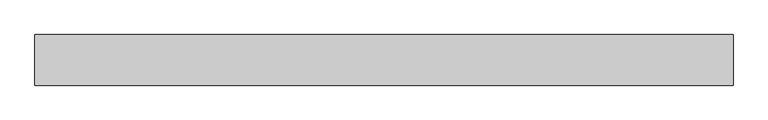
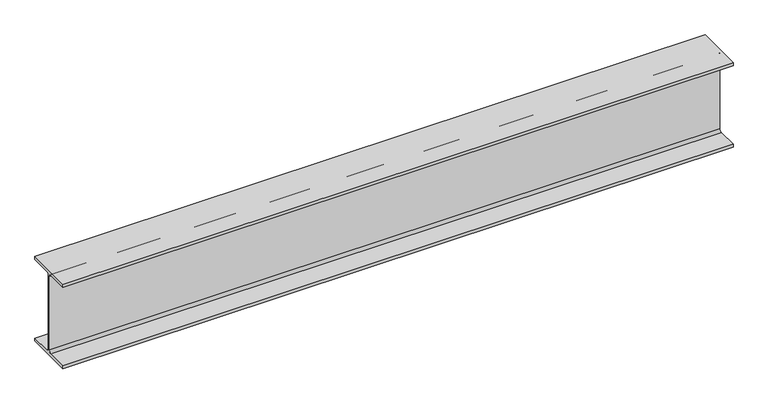
"""IFC4 building model written with IfcOpenShell, lengths in millimetres: beam geometry, Steel Beam_H-KSD3502 : H_SB_ASB_H-200x200x8x12."""

import ifcopenshell
import ifcopenshell.guid

model = None  # the IFC model being written
_history = None  # IfcOwnerHistory: only IFC2X3 demands one
_inside = {}  # id of a spatial element -> (the spatial element, [elements in it])
_under = {}  # id of a project, library or spatial element -> (it, [spatial elements below it])
_declared = {}  # id of a project -> (the project, [libraries it declares])
_typed = {}  # id of a type object -> (the type object, [elements of that type])
_made_of = {}  # id of a material, layer set ... -> (it, [elements and type objects made of it])


def new_model(schema):
    """Start an empty IFC model of exactly this schema.

    Asked for "IFC4X3", IfcOpenShell would pick the latest addendum, in which some entities
    have other attributes; the version numbers below select the first issue.
    IFC2X3 requires an IfcOwnerHistory on every rooted entity: one is made here for all.
    """
    global model, _history
    if schema == "IFC4X3":
        model = ifcopenshell.file(schema_version=(4, 3, 0, 0))
    else:
        model = ifcopenshell.file(schema=schema)
    _inside.clear()
    _under.clear()
    _declared.clear()
    _typed.clear()
    _made_of.clear()
    _history = None
    if model.schema == "IFC2X3":
        org = make("IfcOrganization", Name="unknown")
        user = make(
            "IfcPersonAndOrganization",
            ThePerson=make("IfcPerson", FamilyName="unknown"),
            TheOrganization=org,
        )
        app = make(
            "IfcApplication",
            ApplicationDeveloper=org,
            Version="unknown",
            ApplicationFullName="unknown",
            ApplicationIdentifier="unknown",
        )
        _history = make(
            "IfcOwnerHistory",
            OwningUser=user,
            OwningApplication=app,
            ChangeAction="ADDED",
            CreationDate=0,
        )
    return model


def make(cls, **values):
    """One entity of the class cls with the attributes given. An attribute that is None is left unset."""
    return model.create_entity(
        cls, **{name: value for name, value in values.items() if value is not None}
    )


def rooted(cls, **values):
    """An entity with a GlobalId (a new one), such as an element, a storey or a relation."""
    return make(cls, GlobalId=ifcopenshell.guid.new(), OwnerHistory=_history, **values)


def si_unit(unit_type, name, prefix=None):
    """IfcSIUnit, for example si_unit("LENGTHUNIT", "METRE", prefix="MILLI")."""
    return make("IfcSIUnit", UnitType=unit_type, Prefix=prefix, Name=name)


def assignment(units):
    """IfcUnitAssignment: the units of a project."""
    return None if units is None else make("IfcUnitAssignment", Units=units)


def point(xyz):
    """IfcCartesianPoint."""
    return None if xyz is None else make("IfcCartesianPoint", Coordinates=xyz)


def direction(xyz):
    """IfcDirection."""
    return None if xyz is None else make("IfcDirection", DirectionRatios=xyz)


def frame(location, z_axis=None, x_axis=None):
    """IfcAxis2Placement3D, a coordinate frame: its origin and axes. An axis left out is left unset."""
    return make(
        "IfcAxis2Placement3D",
        Location=point(location),
        Axis=direction(z_axis),
        RefDirection=direction(x_axis),
    )


def frame_2d(location, x_axis=None):
    """IfcAxis2Placement2D, a coordinate frame in the plane: its origin and x axis."""
    return make(
        "IfcAxis2Placement2D", Location=point(location), RefDirection=direction(x_axis)
    )


def origin():
    """The frame at (0, 0, 0) with its axes left unset."""
    return frame((0.0, 0.0, 0.0))


def place(relative_to, where):
    """IfcLocalPlacement: puts the frame where relative to a parent placement (None: the world)."""
    return make(
        "IfcLocalPlacement", PlacementRelTo=relative_to, RelativePlacement=where
    )


def context(
    kind, dimensions, precision=None, world=None, true_north=None, identifier=None
):
    """IfcGeometricRepresentationContext, for example the 3D "Model" context."""
    return make(
        "IfcGeometricRepresentationContext",
        ContextIdentifier=identifier,
        ContextType=kind,
        CoordinateSpaceDimension=dimensions,
        Precision=precision,
        WorldCoordinateSystem=world,
        TrueNorth=true_north,
    )


def project(units=None, contexts=None):
    """IfcProject with its units and contexts."""
    return rooted(
        "IfcProject",
        Name="project",
        RepresentationContexts=contexts,
        UnitsInContext=assignment(units),
    )


def spatial(cls, under=None, at=None, **own):
    """A site, building, storey or space (cls), placed at a placement, below another one or the project."""
    s = rooted(cls, ObjectPlacement=at, **own)
    if under is not None:
        _under.setdefault(under.id(), (under, []))[1].append(s)
    return s


def polyline(points):
    """IfcPolyline through the points."""
    return make("IfcPolyline", Points=[point(p) for p in points])


def circle_curve(where, radius):
    """IfcCircle in the frame where."""
    return make("IfcCircle", Position=where, Radius=radius)


def trimmed(basis, trim1, trim2, sense, master):
    """IfcTrimmedCurve: the piece of a basis curve between two trims."""
    return make(
        "IfcTrimmedCurve",
        BasisCurve=basis,
        Trim1=trim1,
        Trim2=trim2,
        SenseAgreement=sense,
        MasterRepresentation=master,
    )


def segment(curve, same_sense, transition):
    """IfcCompositeCurveSegment."""
    return make(
        "IfcCompositeCurveSegment",
        Transition=transition,
        SameSense=same_sense,
        ParentCurve=curve,
    )


def composite_curve(segments, self_intersect=None):
    """IfcCompositeCurve: segments joined end to end."""
    return make("IfcCompositeCurve", Segments=segments, SelfIntersect=self_intersect)


def outline(outer, holes=None, kind="AREA"):
    """IfcArbitraryClosedProfileDef: a profile drawn as a closed curve; with holes, ...WithVoids."""
    if holes is None:
        return make("IfcArbitraryClosedProfileDef", ProfileType=kind, OuterCurve=outer)
    return make(
        "IfcArbitraryProfileDefWithVoids",
        ProfileType=kind,
        OuterCurve=outer,
        InnerCurves=holes,
    )


def extrude(swept, where, along, depth):
    """IfcExtrudedAreaSolid: the profile swept, set in the frame where, extruded along a direction by depth."""
    return make(
        "IfcExtrudedAreaSolid",
        SweptArea=swept,
        Position=where,
        ExtrudedDirection=direction(along),
        Depth=depth,
    )


def shape(context_of_items, identifier, shape_type, items):
    """IfcShapeRepresentation: the items that make up one representation, for example the "Body"."""
    return make(
        "IfcShapeRepresentation",
        ContextOfItems=context_of_items,
        RepresentationIdentifier=identifier,
        RepresentationType=shape_type,
        Items=items,
    )


def source(mapping_origin, context_of_items, identifier, shape_type, items):
    """IfcRepresentationMap: a shape defined once, which mapped items show again and again."""
    return make(
        "IfcRepresentationMap",
        MappingOrigin=mapping_origin,
        MappedRepresentation=shape(context_of_items, identifier, shape_type, items),
    )


def transform(
    local_origin,
    x_axis=None,
    y_axis=None,
    z_axis=None,
    scale=None,
    scale2=None,
    scale3=None,
    uniform=True,
):
    """IfcCartesianTransformationOperator3D, or its non-uniform kind. x_axis, y_axis, z_axis: its Axis1, 2, 3."""
    if uniform:
        return make(
            "IfcCartesianTransformationOperator3D",
            Axis1=direction(x_axis),
            Axis2=direction(y_axis),
            LocalOrigin=point(local_origin),
            Scale=scale,
            Axis3=direction(z_axis),
        )
    return make(
        "IfcCartesianTransformationOperator3DnonUniform",
        Axis1=direction(x_axis),
        Axis2=direction(y_axis),
        LocalOrigin=point(local_origin),
        Scale=scale,
        Axis3=direction(z_axis),
        Scale2=scale2,
        Scale3=scale3,
    )


def mapped(mapping_source, mapping_target):
    """IfcMappedItem: shows the shape of a source again, moved by a transform."""
    return make(
        "IfcMappedItem", MappingSource=mapping_source, MappingTarget=mapping_target
    )


def made_of(thing, what):
    """Note that an element or type object is made of a material, layer set ...; save() writes the relation."""
    if what is not None:
        _made_of.setdefault(what.id(), (what, []))[1].append(thing)
    return thing


def element(
    cls,
    number,
    at=None,
    inside=None,
    cuts=None,
    type_object=None,
    material=None,
    context=None,
    identifier="Body",
    shape_type=None,
    held_by="IfcProductDefinitionShape",
    body=None,
    shapes=None,
    **own,
):
    """One element of the class cls, such as IfcWall. Its Tag is "e" and its number.

    at: its placement. inside: the storey or other place that contains it. cuts: it is an
    opening in that element (IfcRelVoidsElement). A single representation is given by context,
    identifier, shape_type and body (its items); several are given by shapes. held_by: the class
    of the entity that holds the representations. save() writes the other relations.
    """
    e = rooted(cls, Tag="e%d" % number, ObjectPlacement=at, **own)
    if body is not None:
        shapes = [shape(context, identifier, shape_type, body)]
    if shapes is not None:
        e.Representation = make(held_by, Representations=shapes)
    if inside is not None:
        _inside.setdefault(inside.id(), (inside, []))[1].append(e)
    if cuts is not None:
        rooted(
            "IfcRelVoidsElement", RelatingBuildingElement=cuts, RelatedOpeningElement=e
        )
    if type_object is not None:
        _typed.setdefault(type_object.id(), (type_object, []))[1].append(e)
    return made_of(e, material)


def aggregate(whole, parts):
    """IfcRelAggregates: a whole, such as a stair, and the parts it consists of."""
    return rooted("IfcRelAggregates", RelatingObject=whole, RelatedObjects=parts)


def save(model, path):
    """Write the relations noted so far, then the file.

    IfcRelAggregates (storeys below a building ...), IfcRelContainedInSpatialStructure (elements
    in a storey), IfcRelDefinesByType, IfcRelAssociatesMaterial and IfcRelDeclares: one each for
    every whole, place, type object, material and project.
    """
    for whole, parts in _under.values():
        aggregate(whole, parts)
    for where, things in _inside.values():
        rooted(
            "IfcRelContainedInSpatialStructure",
            RelatedElements=things,
            RelatingStructure=where,
        )
    for kind, things in _typed.values():
        rooted("IfcRelDefinesByType", RelatedObjects=things, RelatingType=kind)
    for what, things in _made_of.values():
        rooted("IfcRelAssociatesMaterial", RelatedObjects=things, RelatingMaterial=what)
    for by, libraries in _declared.values():
        rooted("IfcRelDeclares", RelatingContext=by, RelatedDefinitions=libraries)
    model.write(path)


def beam_8c5619d4(model_context):
    return source(origin(), model_context, "Body", "SweptSolid", [
        extrude(outline(composite_curve([segment(polyline([(82.5, -141.5), (82.5, -151.7), (-82.5, -151.7), (-82.5, -141.5), (-11.9, -141.5)]), True, "CONTINUOUS"), segment(trimmed(circle_curve(frame_2d((-11.9, -132.6)), 8.9), [point((-11.9, -141.5))], [point((-3.0, -132.6))], True, "CARTESIAN"), True, "CONTINUOUS"), segment(polyline([(-3.0, -132.6), (-3.0, 132.6)]), True, "CONTINUOUS"), segment(trimmed(circle_curve(frame_2d((-11.9, 132.6)), 8.9), [point((-3.0, 132.6))], [point((-11.9, 141.5))], True, "CARTESIAN"), True, "CONTINUOUS"), segment(polyline([(-11.9, 141.5), (-82.5, 141.5), (-82.5, 151.7), (82.5, 151.7), (82.5, 141.5), (11.9, 141.5)]), True, "CONTINUOUS"), segment(trimmed(circle_curve(frame_2d((11.9, 132.6)), 8.9), [point((11.9, 141.5))], [point((3.0, 132.6))], True, "CARTESIAN"), True, "CONTINUOUS"), segment(polyline([(3.0, 132.6), (3.0, -132.6)]), True, "CONTINUOUS"), segment(trimmed(circle_curve(frame_2d((11.9, -132.6)), 8.9), [point((3.0, -132.6))], [point((11.9, -141.5))], True, "CARTESIAN"), True, "CONTINUOUS"), segment(polyline([(11.9, -141.5), (82.5, -141.5)]), True, "CONTINUOUS")], self_intersect=False)), frame((-1039.9887612, 0.0, 0.0), z_axis=(1.0, 0.0, 0.0), x_axis=(0.0, 1.0, 0.0)), (0.0, 0.0, 1.0), 2275.0622856),
    ])


if __name__ == "__main__":
    model = new_model("IFC4")
    model_context = context("Model", 3, world=origin())
    ifc_project = project(units=[si_unit("LENGTHUNIT", "METRE", prefix="MILLI")], contexts=[model_context])
    site = spatial("IfcSite", under=ifc_project)
    building = spatial("IfcBuilding", under=site)
    placement = place(None, origin())
    beam_shape = beam_8c5619d4(model_context)
    element("IfcBeam", 1, ObjectType="Steel Beam_H-KSD3502 : H_SB_ASB_H-200x200x8x12", at=placement, inside=building, context=model_context, shape_type="MappedRepresentation", body=[
        mapped(beam_shape, transform((0.0, 0.0, 0.0), x_axis=(1.0, 0.0, 0.0), y_axis=(0.0, 1.0, 0.0), z_axis=(0.0, 0.0, 1.0))),
    ])
    save(model, "model.ifc")

# Revit data of these elements
# Type "Steel Beam_H-KSD3502 : H_SB_ASB_H-200x200x8x12"
#   Width = 20.0 cm
#   Web Thickness = 0.8 cm
#   Web Fillet = 1.3 cm
#   Warping Constant = 141376.0 cm⁶
#   Torsional Moment of Inertia = 26.2485 cm⁴
#   Torsional Modulus = 1.0 cm³
#   Section Area = 63.53 cm²
#   Plastic Modulus weak axis = 244.0 cm³
#   Plastic Modulus strong axis = 525.0 cm³
#   Perimeter = 1.16 m²/m
#   Nominal Weight = 49.90 kgf/m
#   Moment of Inertia weak axis = 1600.00 cm⁴
#   Moment of Inertia strong axis = 4720.00 cm⁴
#   Height = 20.0 cm
#   Flange Thickness = 1.2 cm
#   Elastic Modulus weak axis = 160.0 cm³
#   Elastic Modulus strong axis = 472.0 cm³
#   Centroid Vertical = 10.0 cm
#   Centroid Horizontal = 10.0 cm
#   Length [instance default] = 1.5240 m
#   Structural Material [instance default] = Steel, 45-345
#   Assembly Code = ""
# Element 1 (IfcBeam, "Steel Beam_H-KSD3502 : H_SB_ASB_H-200x200x8x12")
#   Structural Material = none
# Materials
#   "Steel, 45-345": class "Metal", colour RGB 189 187 185, transparency 0, Description = "Steel 345 MPa", Cost = 0
